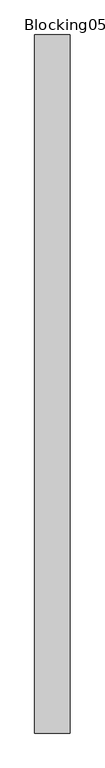
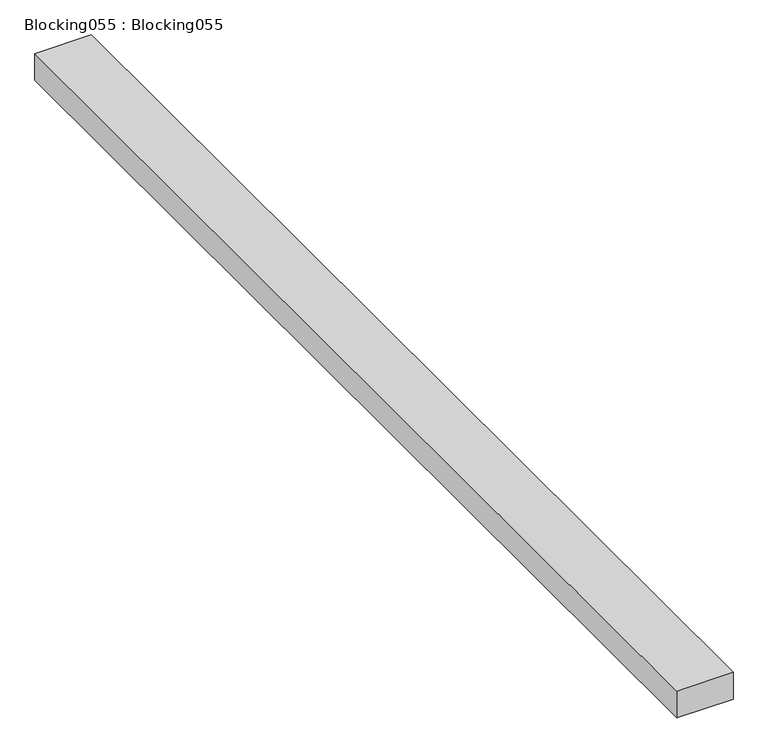
"""IFC4 building model written with IfcOpenShell, lengths in millimetres: proxy geometry, Blocking055 : Blocking055."""

from ifc_helpers import new_model, si_unit, frame, origin, place, context, project, spatial, polyline, outline, extrude, source, transform, mapped, element, save


def blocking055_blocking055_44976e41(model_context):
    return source(origin(), model_context, "Body", "SweptSolid", [
        extrude(outline(polyline([(-9298.3737014, 7982.1531721), (-9399.9737014, 7982.1531721), (-9399.9737014, 9982.1531721), (-9298.3737014, 9982.1531721), (-9298.3737014, 7982.1531721)])), frame((0.0, 0.0, 40106.3460083), z_axis=(0.0, 0.0, 1.0), x_axis=(1.0, 0.0, 0.0)), (0.0, 0.0, 1.0), 50.8),
    ])


if __name__ == "__main__":
    model = new_model("IFC4")
    model_context = context("Model", 3, world=origin())
    ifc_project = project(units=[si_unit("LENGTHUNIT", "METRE", prefix="MILLI")], contexts=[model_context])
    site = spatial("IfcSite", under=ifc_project)
    building = spatial("IfcBuilding", under=site)
    placement = place(None, origin())
    blocking055_blocking055_shape = blocking055_blocking055_44976e41(model_context)
    element("IfcBuildingElementProxy", 1, Name="Blocking055 : Blocking055", ObjectType="Blocking055 : Blocking055", at=placement, inside=building, context=model_context, shape_type="MappedRepresentation", body=[
        mapped(blocking055_blocking055_shape, transform((0.0, 0.0, 0.0), x_axis=(1.0, 0.0, 0.0), y_axis=(0.0, 1.0, 0.0), z_axis=(0.0, 0.0, 1.0))),
    ])
    save(model, "model.ifc")

# Revit data of these elements
# Type "Blocking055 : Blocking055"
#   NameOverride = "Blocking055"
# Element 1 (IfcBuildingElementProxy, "Blocking055 : Blocking055")
#   Materials on its faces: "WOOD BLOCKING AS REQUIRED"
# Materials
#   "WOOD BLOCKING AS REQUIRED": class "Unassigned", colour RGB 166 124 85, transparency 0, Cost = 0
